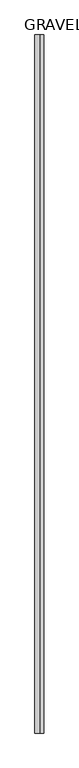
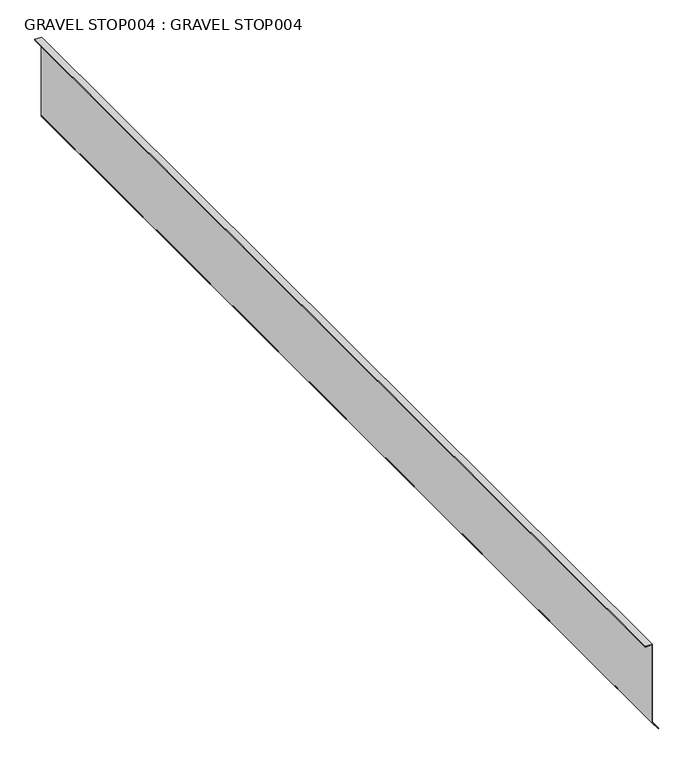
"""IFC4 building model written with IfcOpenShell, lengths in millimetres: proxy geometry, GRAVEL STOP004 : GRAVEL STOP004."""

from ifc_helpers import new_model, si_unit, frame, origin, place, context, project, spatial, polyline, outline, extrude, source, transform, mapped, element, save


def gravel_stop004_gravel_stop004_78d96abb(model_context):
    return source(origin(), model_context, "Body", "SweptSolid", [
        extrude(outline(polyline([(40082.2407116, -4352.793241), (40097.9858473, -4365.3568119), (40254.7357103, -4365.3568119), (40254.7357103, -4378.5358417), (40253.3245993, -4378.5358417), (40253.3245993, -4366.7679229), (40097.4918556, -4366.7679229), (40081.3605882, -4353.8962446), (40082.2407116, -4352.793241)])), frame((0.0, -1065.5906573, 0.0), z_axis=(0.0, 1.0, 0.0), x_axis=(0.0, 0.0, 1.0)), (0.0, 0.0, 1.0), 2000.25),
    ])


if __name__ == "__main__":
    model = new_model("IFC4")
    model_context = context("Model", 3, world=origin())
    ifc_project = project(units=[si_unit("LENGTHUNIT", "METRE", prefix="MILLI")], contexts=[model_context])
    site = spatial("IfcSite", under=ifc_project)
    building = spatial("IfcBuilding", under=site)
    placement = place(None, origin())
    gravel_stop004_gravel_stop004_shape = gravel_stop004_gravel_stop004_78d96abb(model_context)
    element("IfcBuildingElementProxy", 1, Name="GRAVEL STOP004 : GRAVEL STOP004", ObjectType="GRAVEL STOP004 : GRAVEL STOP004", at=placement, inside=building, context=model_context, shape_type="MappedRepresentation", body=[
        mapped(gravel_stop004_gravel_stop004_shape, transform((0.0, 0.0, 0.0), x_axis=(1.0, 0.0, 0.0), y_axis=(0.0, 1.0, 0.0), z_axis=(0.0, 0.0, 1.0))),
    ])
    save(model, "model.ifc")

# Revit data of these elements
# Type "GRAVEL STOP004 : GRAVEL STOP004"
#   NameOverride = "GRAVEL STOP004"
# Element 1 (IfcBuildingElementProxy, "GRAVEL STOP004 : GRAVEL STOP004")
#   Materials on its faces: "GRAVEL STOP REQUIRED WITH GRAVEL SURFACE SYSTEMS"
# Materials
#   "GRAVEL STOP REQUIRED WITH GRAVEL SURFACE SYSTEMS": class "Unassigned", colour RGB 170 170 127, transparency 0
